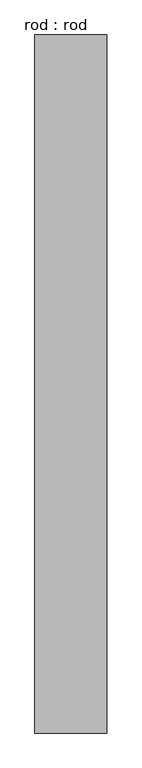
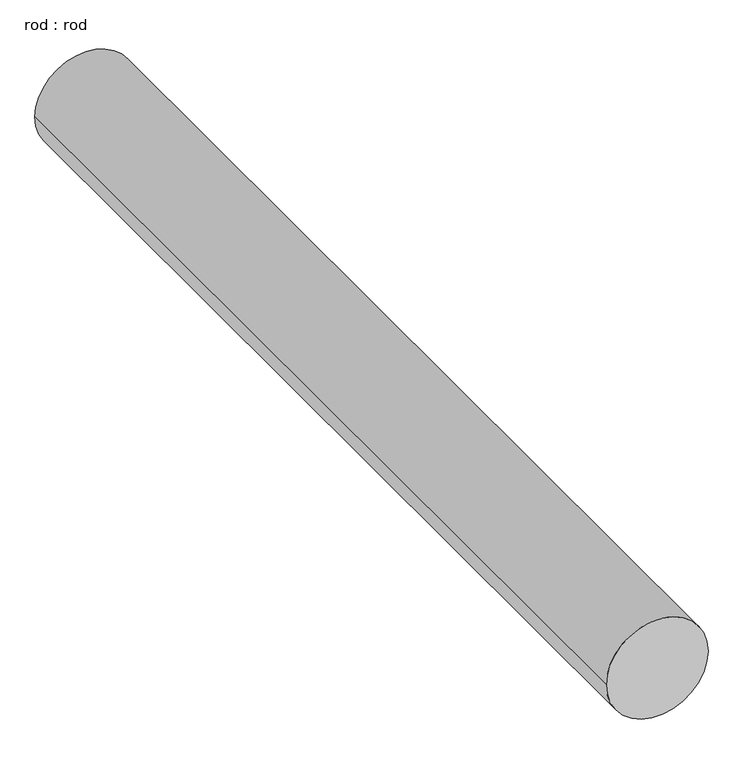
"""IFC4 building model written with IfcOpenShell, lengths in millimetres: proxy geometry, rod : rod."""

from ifc_helpers import new_model, si_unit, point, frame, frame_2d, origin, place, context, project, spatial, circle_curve, trimmed, segment, composite_curve, outline, extrude, source, transform, mapped, element, save


def rod_rod_3d32d602(model_context):
    return source(origin(), model_context, "Body", "SweptSolid", [
        extrude(outline(composite_curve([segment(trimmed(circle_curve(frame_2d((0.0108462, 0.0)), 200.0), [point((0.0108462, 200.0))], [point((0.0108462, -200.0))], False, "CARTESIAN"), True, "CONTINUOUS"), segment(trimmed(circle_curve(frame_2d((0.0108462, 0.0)), 200.0), [point((0.0108462, -200.0))], [point((0.0108462, 200.0))], False, "CARTESIAN"), True, "CONTINUOUS")], self_intersect=False)), frame((0.0, 2151.9668448, 0.0), z_axis=(0.0, 1.0, 0.0), x_axis=(0.0, 0.0, 1.0)), (0.0, 0.0, 1.0), 3881.5235411),
    ])


if __name__ == "__main__":
    model = new_model("IFC4")
    model_context = context("Model", 3, world=origin())
    ifc_project = project(units=[si_unit("LENGTHUNIT", "METRE", prefix="MILLI")], contexts=[model_context])
    site = spatial("IfcSite", under=ifc_project)
    building = spatial("IfcBuilding", under=site)
    placement = place(None, origin())
    rod_rod_shape = rod_rod_3d32d602(model_context)
    element("IfcBuildingElementProxy", 1, Name="rod : rod", ObjectType="rod : rod", at=placement, inside=building, context=model_context, shape_type="MappedRepresentation", body=[
        mapped(rod_rod_shape, transform((0.0, 0.0, 0.0), x_axis=(1.0, 0.0, 0.0), y_axis=(0.0, 1.0, 0.0), z_axis=(0.0, 0.0, 1.0))),
    ])
    save(model, "model.ifc")

# Revit data of these elements
# Type "rod : rod"
#   Default Elevation = 0
